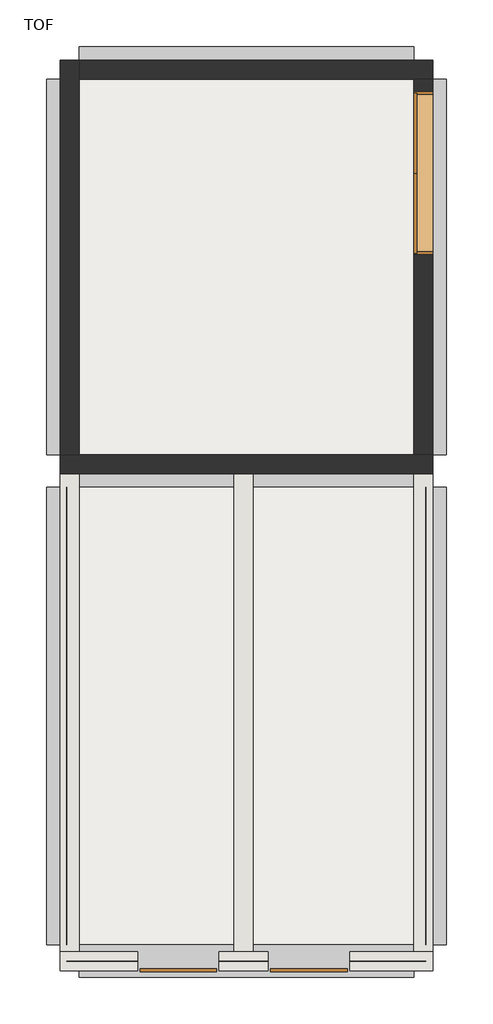
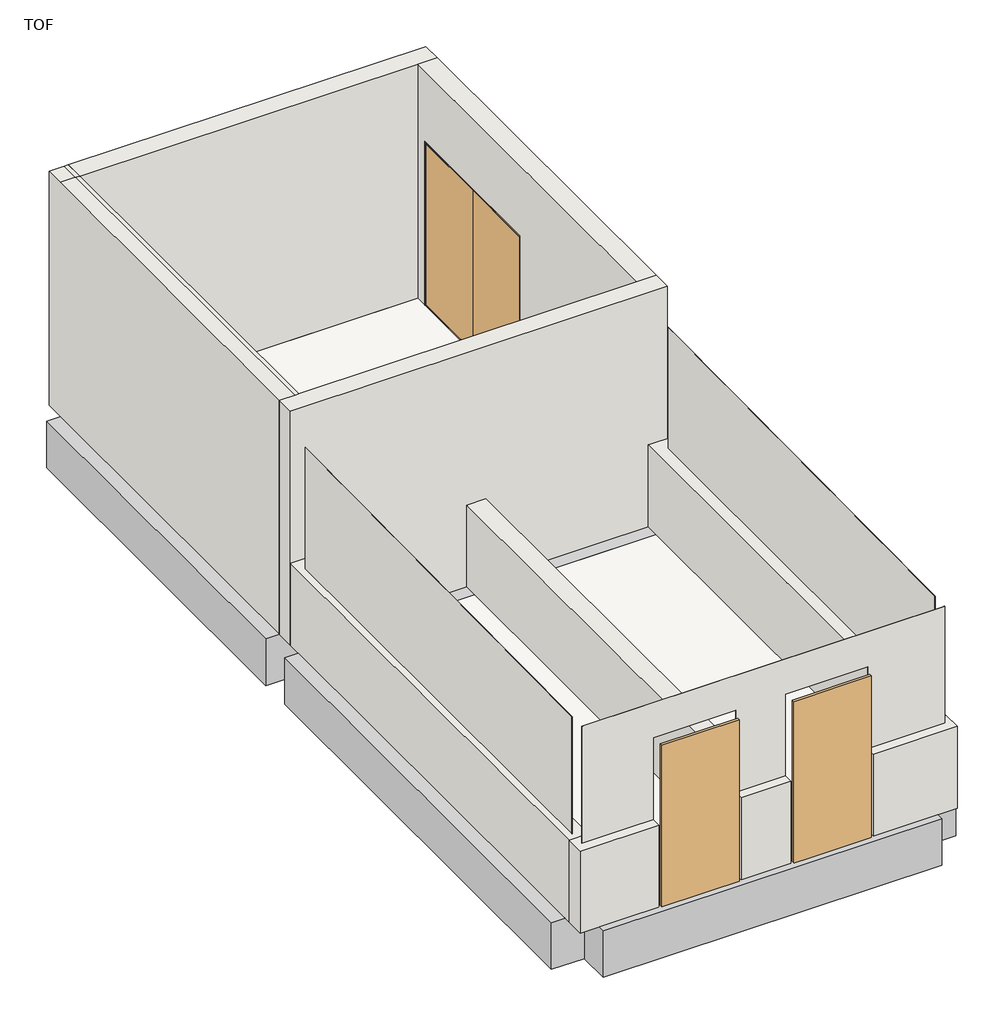
# One storey: 11 walls, 7 beams, 3 doors, 2 slabs.
# Revit data of these elements (continued)
# Room, not placed, phase "New Construction", upper offset 0.000 mm, lower offset 0.000 mm (continued)
#   Base Finish-2 = ""
#   Base Finish-3 = "Glazed Ceramic Tile"
#   Base Finish-4 = ""
#   Wall Finish-1 = "Glazed Ceramic Tile (<=2100) / Acrylic Emulsion Paint (>2100) on Cement Plaster"
#   Wall Finish-2 = "H=2100"
#   Ceiling Finish Style Name = "Suspended Moisture Resistant Tiled Ceiling (T-Bar)"
#   Ceiling Finish Ref. = "600x600\nT bar"
#   Ceiling-Base Material = "Concrete Slab"
#   Ceiling Finish-1 = ""
#   Ceiling Finish-2 = ""
#   Ceiling Finish-3 = "Moisture Resistant Tiled Ceiling System (T-Bar)"
#   Ceiling Finish-4 = ""
#   H_Room L = 3400.000 mm
#   H_Room W = 3000.000 mm
#   H_Room H or CH = 7300.000 mm
#   Floor Finish Style No = F31A
#   Base Finish Style No = B32
#   Wall Finish Style No = W32B-1
#   Ceiling Finish Style No = C96A
# Room, not placed, phase "New Construction", upper offset 0.000 mm, lower offset 0.000 mm
#   Comments = ""
#   Number = "110"
#   Name = "ABLUTIONS"
#   Floor Finish Style Name = "Non-Slip Unglazed Ceramic Tile on Screed + Liquid Waterproofing"
#   Floor Finish Ref. = ""
#   Floor-Base Material = "Concrete Slab"
#   Floor Finish-1 = "Screed"
#   Floor Finish-2 = "Liquid Waterproofing"
#   Floor Finish-3 = "Ceramic Tile"
#   Floor Finish-4 = ""
#   Base Finish Style Name = "Coved Ceramic Tile"
#   Base Finish Ref. = ""
#   Base-Base Material = "Concrete Wall\n/ Masonry Wall"
#   Base Finish-1 = ""
#   Base Finish-2 = ""
#   Base Finish-3 = "Glazed Ceramic Tile"
#   Base Finish-4 = ""
#   Wall Finish-1 = "Glazed Ceramic Tile (<=2100) / Acrylic Emulsion Paint (>2100) on Cement Plaster"
#   Wall Finish-2 = "H=2100"
#   Ceiling Finish Style Name = "Suspended Moisture Resistant Tiled Ceiling (T-Bar)"
#   Ceiling Finish Ref. = "600x600\nT bar"
#   Ceiling-Base Material = "Concrete Slab"
#   Ceiling Finish-1 = ""
#   Ceiling Finish-2 = ""
#   Ceiling Finish-3 = "Moisture Resistant Tiled Ceiling System (T-Bar)"
#   Ceiling Finish-4 = ""
#   H_Room L = 3400.000 mm
#   H_Room W = 2200.000 mm
#   H_Room H or CH = 6300.000 mm
#   Floor Finish Style No = F31B
#   Base Finish Style No = B32
#   Wall Finish Style No = W32B-1
#   Ceiling Finish Style No = C96A
# Room, not placed, phase "New Construction", upper offset 0.000 mm, lower offset 0.000 mm
#   Comments = ""
#   Number = "112"
#   Name = "ELECTRICAL ROOM(SS08) [F-1]"
#   Floor Finish Style Name = "Non-Slip Epoxy Paint on Screed"
#   Floor Finish Ref. = ""
#   Floor-Base Material = "Concrete Slab"
#   Floor Finish-1 = "Screed"
#   Floor Finish-2 = ""
#   Floor Finish-3 = "Epoxy Paint"
#   Floor Finish-4 = ""
#   Base Finish Style Name = "Epoxy Paint"
#   Base Finish Ref. = ""
#   Base-Base Material = "Concrete Wall\n/ Masonry Wall \n/ Dry Wall"
#   Base Finish-1 = ""
#   Base Finish-2 = ""
#   Base Finish-3 = "Epoxy Paint"
#   Base Finish-4 = ""
#   Wall Finish-1 = "Acrylic Emulsion Paint on Cement Plaster"
#   Wall Finish-2 = "T13 Plaster"
#   Ceiling Finish Style Name = "Acrylic Emulsion Paint on Fair Faced Concrete"
#   Ceiling Finish Ref. = ""
#   Ceiling-Base Material = "Concrete Slab"
#   Ceiling Finish-1 = ""
#   Ceiling Finish-2 = ""
#   Ceiling Finish-3 = "Acrylic Emulsion Paint"
#   Ceiling Finish-4 = ""
#   H_Room L = 11700.000 mm
#   H_Room W = 18000.000 mm
#   H_Room H or CH = 7300.000 mm
#   Floor Finish Style No = F06B
#   Base Finish Style No = B03
#   Wall Finish Style No = W01B
#   Ceiling Finish Style No = C01
# Room, not placed, phase "New Construction", upper offset 0.000 mm, lower offset 0.000 mm
#   Comments = ""
#   Number = "114"
#   Name = "BATTERY ROOM [F-1]"
#   Floor Finish Style Name = "Acid Resistant Ceramic Tile on Screed"
#   Floor Finish Ref. = ""
#   Floor-Base Material = "Concrete Slab"
#   Floor Finish-1 = "Screed"
#   Floor Finish-2 = ""
#   Floor Finish-3 = "Acid/Alkaline Resistant Tile"
#   Floor Finish-4 = ""
#   Base Finish Style Name = "Acid Resistant Ceramic Tile"
#   Base Finish Ref. = ""
#   Base-Base Material = "Concrete Wall\n/ Masonry Wall"
#   Base Finish-1 = ""
#   Base Finish-2 = ""
#   Base Finish-3 = "Acid/Alkaline Resistant Tile"
#   Base Finish-4 = ""
#   Wall Finish-1 = "Acid Resistant Paint on Cement Plaster"
#   Wall Finish-2 = "T13 Plaster"
#   Ceiling Finish Style Name = "Acrylic Emulsion Paint on Fair Faced Concrete"
#   Ceiling Finish Ref. = ""
#   Ceiling-Base Material = "Concrete Slab"
#   Ceiling Finish-1 = ""
#   Ceiling Finish-2 = ""
#   Ceiling Finish-3 = "Acrylic Emulsion Paint"
#   Ceiling Finish-4 = ""
#   H_Room L = 7800.000 mm
#   H_Room W = 8300.000 mm
#   H_Room H or CH = 7300.000 mm
#   Floor Finish Style No = F32
#   Base Finish Style No = B33
#   Wall Finish Style No = W04B
#   Ceiling Finish Style No = C01
# Room, not placed, phase "New Construction", upper offset 0.000 mm, lower offset 0.000 mm
#   Comments = ""
#   Number = "118"
#   Name = "DRIVERS LOUNGE"
#   Floor Finish Style Name = "Vinyl Tile on Screed"
#   Floor Finish Ref. = ""
#   Floor-Base Material = "Concrete Slab"
#   Floor Finish-1 = "Screed"
#   Floor Finish-2 = ""
#   Floor Finish-3 = "Vinyl Tile"
#   Floor Finish-4 = ""
#   Base Finish Style Name = "Coved Vinyl Tile"
#   Base Finish Ref. = ""
#   Base-Base Material = "Concrete Wall\n/ Masonry Wall"
#   Base Finish-1 = ""
#   Base Finish-2 = ""
#   Base Finish-3 = "Vinyl Tile"
#   Base Finish-4 = ""
#   Wall Finish-1 = "Acrylic Emulsion Paint on Cement Plaster"
#   Wall Finish-2 = "T13 Plaster"
#   Ceiling Finish Style Name = "Suspended Acoustic Tiled Ceiling (T-Bar)"
#   Ceiling Finish Ref. = "600x600\nT Bar"
#   Ceiling-Base Material = "Concrete Slab"
#   Ceiling Finish-1 = ""
#   Ceiling Finish-2 = ""
#   Ceiling Finish-3 = "Acoustic Tiled Ceiling System (T-Bar)"
#   Ceiling Finish-4 = ""
#   H_Room L = 7800.000 mm
#   H_Room W = 4500.000 mm
#   H_Room H or CH = 6300.000 mm
#   Floor Finish Style No = F34A
#   Base Finish Style No = B35A
#   Wall Finish Style No = W01B
#   Ceiling Finish Style No = C95A
# Room, not placed, phase "New Construction", upper offset 0.000 mm, lower offset 0.000 mm
#   Comments = ""
#   Number = "122"
#   Name = "TOILETS"
#   Floor Finish Style Name = "Non-Slip Unglazed Ceramic Tile on Screed + Liquid Waterproofing"
#   Floor Finish Ref. = ""
#   Floor-Base Material = "Concrete Slab"
#   Floor Finish-1 = "Screed"
#   Floor Finish-2 = "Liquid Waterproofing"
#   Floor Finish-3 = "Ceramic Tile"
#   Floor Finish-4 = ""
#   Base Finish Style Name = "Coved Ceramic Tile"
#   Base Finish Ref. = ""
#   Base-Base Material = "Concrete Wall\n/ Masonry Wall"
#   Base Finish-1 = ""
#   Base Finish-2 = ""
#   Base Finish-3 = "Glazed Ceramic Tile"
#   Base Finish-4 = ""
#   Wall Finish-1 = "Glazed Ceramic Tile (<=2100) / Acrylic Emulsion Paint (>2100) on Cement Plaster"
#   Wall Finish-2 = "H=2100"
#   Ceiling Finish Style Name = "Suspended Moisture Resistant Tiled Ceiling (T-Bar)"
#   Ceiling Finish Ref. = "600x600\nT bar"
#   Ceiling-Base Material = "Concrete Slab"
#   Ceiling Finish-1 = ""
#   Ceiling Finish-2 = ""
#   Ceiling Finish-3 = "Moisture Resistant Tiled Ceiling System (T-Bar)"
#   Ceiling Finish-4 = ""
#   H_Room L = 4400.000 mm
#   H_Room W = 4300.000 mm
#   H_Room H or CH = 7300.000 mm
#   Floor Finish Style No = F31B
#   Base Finish Style No = B32
#   Wall Finish Style No = W32B-1
#   Ceiling Finish Style No = C96A
# Room, not placed, phase "New Construction", upper offset 0.000 mm, lower offset 0.000 mm
#   Comments = ""
#   Number = "119"
#   Name = "AIR LOCK"
#   Floor Finish Style Name = "Vinyl Tile on Screed + Matwell"
#   Floor-Base Material = "Concrete Slab"
#   Floor Finish-1 = "Screed"
#   Floor Finish-3 = "Vinyl Tile"
#   Floor Finish-4 = "Matwell"
#   Base Finish Style Name = "Coved Vinyl Tile"
#   Base Finish Ref. = ""
#   Base-Base Material = "Concrete Wall\n/ Masonry Wall"
#   Base Finish-1 = ""
#   Base Finish-2 = ""
#   Base Finish-3 = "Vinyl Tile"
#   Base Finish-4 = ""
#   Wall Finish-1 = "Acrylic Emulsion Paint on Cement Plaster"
#   Wall Finish-2 = "T13 Plaster"
#   Ceiling Finish Style Name = "Suspended Acoustic Tiled Ceiling (T-Bar)"
#   Ceiling Finish Ref. = "600x600\nT Bar"
#   Ceiling-Base Material = "Concrete Slab"
#   Ceiling Finish-1 = ""
#   Ceiling Finish-2 = ""
#   Ceiling Finish-3 = "Acoustic Tiled Ceiling System (T-Bar)"
#   Ceiling Finish-4 = ""
#   H_Room L = 2700.000 mm
#   H_Room W = 2600.000 mm
#   H_Room H or CH = 6300.000 mm
#   Floor Finish Style No = F34A-1
#   Base Finish Style No = B35A
#   Wall Finish Style No = W01B
#   Ceiling Finish Style No = C95A
# Room, not placed, phase "New Construction", upper offset 0.000 mm, lower offset 0.000 mm
#   Comments = ""
#   Number = "124"
#   Name = "STORE"
#   Floor Finish Style Name = "Vinyl Tile on Screed"
#   Floor Finish Ref. = ""
#   Floor-Base Material = "Concrete Slab"
#   Floor Finish-1 = "Screed"
#   Floor Finish-2 = ""
#   Floor Finish-3 = "Vinyl Tile"
#   Floor Finish-4 = ""
#   Base Finish Style Name = "Coved Vinyl Tile"
#   Base Finish Ref. = ""
#   Base-Base Material = "Concrete Wall\n/ Masonry Wall"
#   Base Finish-1 = ""
#   Base Finish-2 = ""
#   Base Finish-3 = "Vinyl Tile"
#   Base Finish-4 = ""
#   Wall Finish-1 = "Acrylic Emulsion Paint on Cement Plaster"
#   Wall Finish-2 = "T13 Plaster"
#   Ceiling Finish Style Name = "Suspended Acoustic Tiled Ceiling (T-Bar)"
#   Ceiling Finish Ref. = "600x600\nT Bar"
#   Ceiling-Base Material = "Concrete Slab"
#   Ceiling Finish-1 = ""
#   Ceiling Finish-2 = ""
#   Ceiling Finish-3 = "Acoustic Tiled Ceiling System (T-Bar)"
#   Ceiling Finish-4 = ""
#   H_Room L = 4400.000 mm
#   H_Room W = 3400.000 mm
#   H_Room H or CH = 7300.000 mm
#   Floor Finish Style No = F34A
#   Base Finish Style No = B35A
#   Wall Finish Style No = W01B
#   Ceiling Finish Style No = C95A
# Room, not placed, phase "New Construction", upper offset 0.000 mm, lower offset 0.000 mm
#   Comments = ""
#   Number = "125"
#   Name = "MAINTENANCE WORKSHOP [F-1]"
#   Floor Finish Style Name = "Non-Slip Epoxy Paint on Steel Trowel Finish"
#   Floor Finish Ref. = ""
#   Floor-Base Material = "Concrete Slab"
#   Floor Finish-1 = "Steel Trowel Finish"
#   Floor Finish-2 = ""
#   Floor Finish-3 = "Epoxy Paint"
#   Floor Finish-4 = ""
#   Base Finish Style Name = "Epoxy Paint"
#   Base Finish Ref. = ""
#   Base-Base Material = "Concrete Wall\n/ Masonry Wall \n/ Dry Wall"
#   Base Finish-1 = ""
#   Base Finish-2 = ""
#   Base Finish-3 = "Epoxy Paint"
#   Base Finish-4 = ""
#   Wall Finish-1 = "Acrylic Emulsion Paint on Cement Plaster"
#   Wall Finish-2 = "T13 Plaster"
#   Ceiling Finish Style Name = "Acrylic Emulsion Paint on Fair Faced Concrete"
#   Ceiling Finish Ref. = ""
#   Ceiling-Base Material = "Concrete Slab"
#   Ceiling Finish-1 = ""
#   Ceiling Finish-2 = ""
#   Ceiling Finish-3 = "Acrylic Emulsion Paint"
#   Ceiling Finish-4 = ""
#   H_Room L = 7800.000 mm
#   H_Room W = 7700.000 mm
#   H_Room H or CH = 7300.000 mm
#   Floor Finish Style No = F06A
#   Base Finish Style No = B03
#   Wall Finish Style No = W01B
#   Ceiling Finish Style No = C01
# Room, not placed, phase "New Construction", upper offset 0.000 mm, lower offset 0.000 mm
#   Comments = ""
#   Number = "120"
#   Name = "CORRIDOR"
#   Floor Finish Style Name = "Vinyl Tile on Screed"
#   Floor Finish Ref. = ""
#   Floor-Base Material = "Concrete Slab"
#   Floor Finish-1 = "Screed"
#   Floor Finish-2 = ""
#   Floor Finish-3 = "Vinyl Tile"
#   Floor Finish-4 = ""
#   Base Finish Style Name = "Coved Vinyl Tile"
#   Base Finish Ref. = ""
#   Base-Base Material = "Concrete Wall\n/ Masonry Wall"
#   Base Finish-1 = ""
#   Base Finish-2 = ""
#   Base Finish-3 = "Vinyl Tile"
#   Base Finish-4 = ""
#   Wall Finish-1 = "Acrylic Emulsion Paint on Cement Plaster"
#   Wall Finish-2 = "T13 Plaster"
#   Ceiling Finish Style Name = "Suspended Acoustic Tiled Ceiling (T-Bar)"
#   Ceiling Finish Ref. = "600x600\nT Bar"
#   Ceiling-Base Material = "Concrete Slab"
#   Ceiling Finish-1 = ""
#   Ceiling Finish-2 = ""
#   Ceiling Finish-3 = "Acoustic Tiled Ceiling System (T-Bar)"
#   Ceiling Finish-4 = ""
#   H_Room L = 7700.000 mm
#   H_Room W = 14400.000 mm
#   H_Room H or CH = 3600.000 mm
#   Floor Finish Style No = F34A
#   Base Finish Style No = B35A
#   Wall Finish Style No = W01B
#   Ceiling Finish Style No = C95A
# Room, not placed, phase "New Construction", upper offset 0.000 mm, lower offset 0.000 mm
#   Comments = ""
#   Number = "123"
#   Name = "STORE"
#   Floor Finish Style Name = "Vinyl Tile on Screed"
#   Floor Finish Ref. = ""
#   Floor-Base Material = "Concrete Slab"
#   Floor Finish-1 = "Screed"
#   Floor Finish-2 = ""
#   Floor Finish-3 = "Vinyl Tile"
#   Floor Finish-4 = ""
#   Base Finish Style Name = "Coved Vinyl Tile"
#   Base Finish Ref. = ""
#   Base-Base Material = "Concrete Wall\n/ Masonry Wall"
#   Base Finish-1 = ""
#   Base Finish-2 = ""
#   Base Finish-3 = "Vinyl Tile"
#   Base Finish-4 = ""
#   Wall Finish-1 = "Acrylic Emulsion Paint on Cement Plaster"
#   Wall Finish-2 = "T13 Plaster"
#   Ceiling Finish Style Name = "Suspended Acoustic Tiled Ceiling (T-Bar)"
#   Ceiling Finish Ref. = "600x600\nT Bar"
#   Ceiling-Base Material = "Concrete Slab"
#   Ceiling Finish-1 = ""
#   Ceiling Finish-2 = ""
#   Ceiling Finish-3 = "Acoustic Tiled Ceiling System (T-Bar)"
#   Ceiling Finish-4 = ""
#   H_Room L = 1800.000 mm
#   H_Room W = 3400.000 mm
#   H_Room H or CH = 3700.000 mm
#   Floor Finish Style No = F34A
#   Base Finish Style No = B35A
#   Wall Finish Style No = W01B
#   Ceiling Finish Style No = C95A
# Room, not placed, phase "New Construction", upper offset 0.000 mm, lower offset 0.000 mm
#   Comments = ""
#   Number = "107"
#   Name = "CORRIDOR"
#   Floor Finish Style Name = "Vinyl Tile on Screed"
#   Floor Finish Ref. = ""
#   Floor-Base Material = "Concrete Slab"
#   Floor Finish-1 = "Screed"
#   Floor Finish-2 = ""
#   Floor Finish-3 = "Vinyl Tile"
#   Floor Finish-4 = ""
#   Base Finish Style Name = "Coved Vinyl Tile"
#   Base Finish Ref. = ""
#   Base-Base Material = "Concrete Wall\n/ Masonry Wall"
#   Base Finish-1 = ""
#   Base Finish-2 = ""
#   Base Finish-3 = "Vinyl Tile"
#   Base Finish-4 = ""
#   Wall Finish-1 = "Acrylic Emulsion Paint on Cement Plaster"
#   Wall Finish-2 = "T13 Plaster"
#   Ceiling Finish Style Name = "Suspended Acoustic Tiled Ceiling (T-Bar)"
#   Ceiling Finish Ref. = "600x600\nT Bar"
#   Ceiling-Base Material = "Concrete Slab"
#   Ceiling Finish-1 = ""
#   Ceiling Finish-2 = ""
#   Ceiling Finish-3 = "Acoustic Tiled Ceiling System (T-Bar)"
#   Ceiling Finish-4 = ""
#   H_Room L = 10500.000 mm
#   H_Room W = 3800.000 mm
#   H_Room H or CH = 3700.000 mm
#   Floor Finish Style No = F34A
#   Base Finish Style No = B35A
#   Wall Finish Style No = W01B
#   Ceiling Finish Style No = C95A
